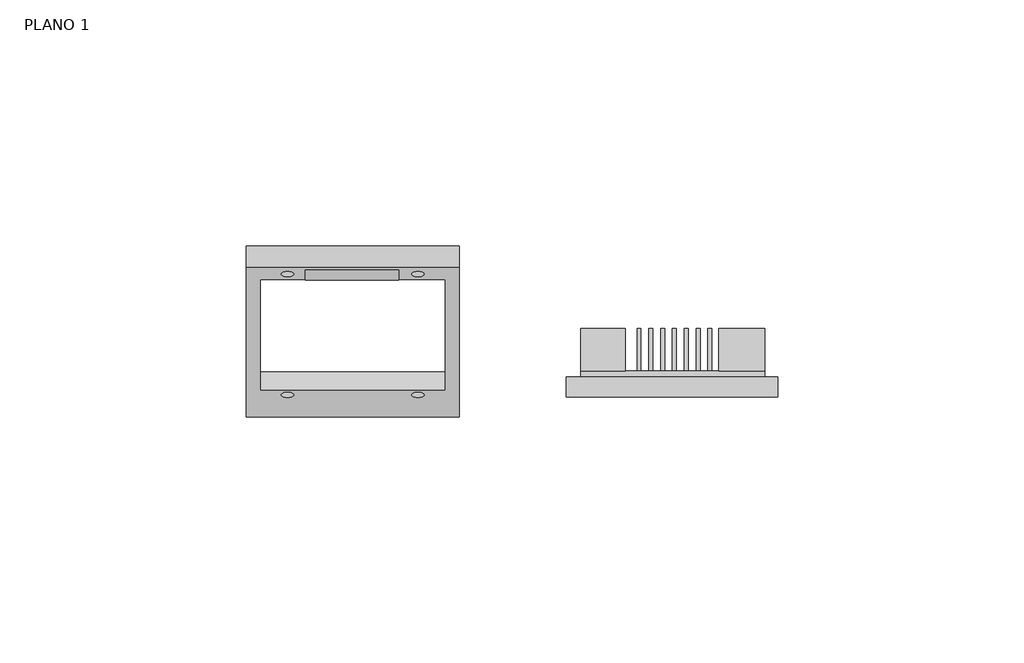
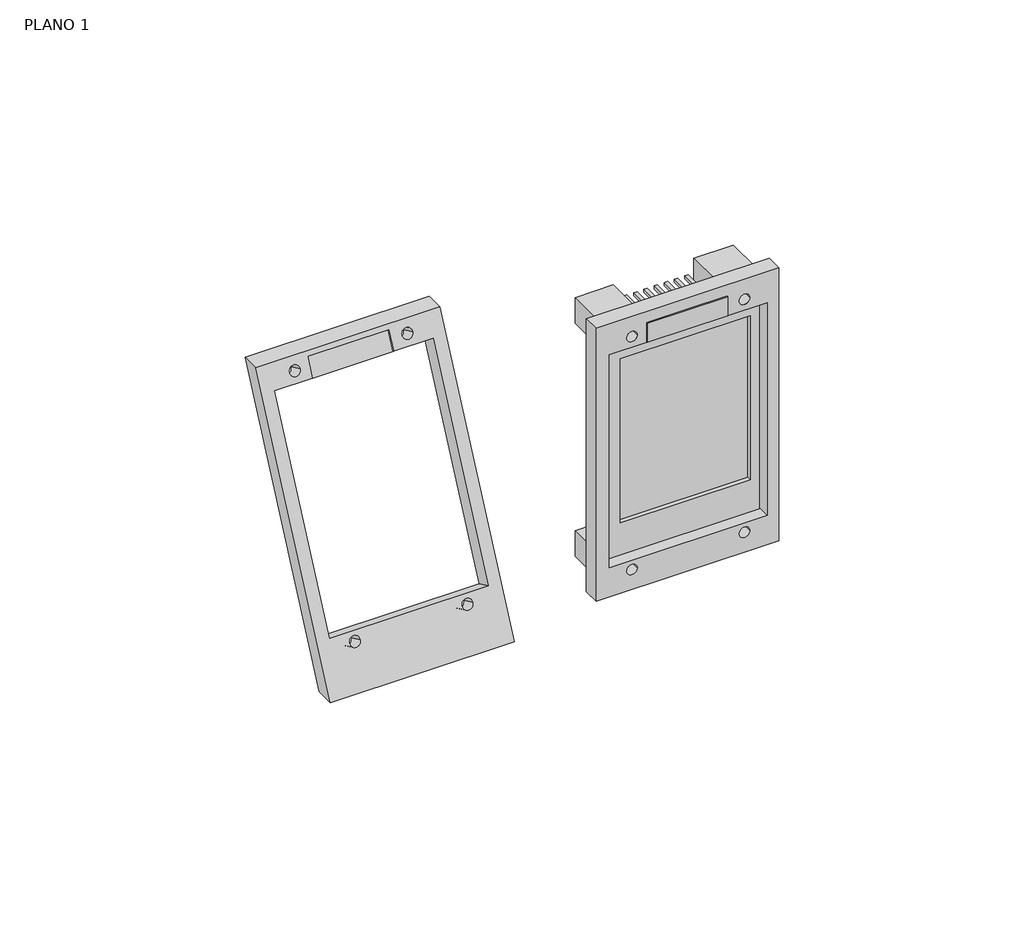
# One storey: 3 furniture elements, 2 proxies.
"""IFC4 building model written with IfcOpenShell, lengths in millimetres."""

import ifcopenshell
import ifcopenshell.guid

model = None  # the IFC model being written
_history = None  # IfcOwnerHistory: only IFC2X3 demands one
_inside = {}  # id of a spatial element -> (the spatial element, [elements in it])
_under = {}  # id of a project, library or spatial element -> (it, [spatial elements below it])
_declared = {}  # id of a project -> (the project, [libraries it declares])
_typed = {}  # id of a type object -> (the type object, [elements of that type])
_made_of = {}  # id of a material, layer set ... -> (it, [elements and type objects made of it])


def new_model(schema):
    """Start an empty IFC model of exactly this schema.

    Asked for "IFC4X3", IfcOpenShell would pick the latest addendum, in which some entities
    have other attributes; the version numbers below select the first issue.
    IFC2X3 requires an IfcOwnerHistory on every rooted entity: one is made here for all.
    """
    global model, _history
    if schema == "IFC4X3":
        model = ifcopenshell.file(schema_version=(4, 3, 0, 0))
    else:
        model = ifcopenshell.file(schema=schema)
    _inside.clear()
    _under.clear()
    _declared.clear()
    _typed.clear()
    _made_of.clear()
    _history = None
    if model.schema == "IFC2X3":
        org = make("IfcOrganization", Name="unknown")
        user = make(
            "IfcPersonAndOrganization",
            ThePerson=make("IfcPerson", FamilyName="unknown"),
            TheOrganization=org,
        )
        app = make(
            "IfcApplication",
            ApplicationDeveloper=org,
            Version="unknown",
            ApplicationFullName="unknown",
            ApplicationIdentifier="unknown",
        )
        _history = make(
            "IfcOwnerHistory",
            OwningUser=user,
            OwningApplication=app,
            ChangeAction="ADDED",
            CreationDate=0,
        )
    return model


def make(cls, **values):
    """One entity of the class cls with the attributes given. An attribute that is None is left unset."""
    return model.create_entity(
        cls, **{name: value for name, value in values.items() if value is not None}
    )


def rooted(cls, **values):
    """An entity with a GlobalId (a new one), such as an element, a storey or a relation."""
    return make(cls, GlobalId=ifcopenshell.guid.new(), OwnerHistory=_history, **values)


def si_unit(unit_type, name, prefix=None):
    """IfcSIUnit, for example si_unit("LENGTHUNIT", "METRE", prefix="MILLI")."""
    return make("IfcSIUnit", UnitType=unit_type, Prefix=prefix, Name=name)


def assignment(units):
    """IfcUnitAssignment: the units of a project."""
    return None if units is None else make("IfcUnitAssignment", Units=units)


def point(xyz):
    """IfcCartesianPoint."""
    return None if xyz is None else make("IfcCartesianPoint", Coordinates=xyz)


def direction(xyz):
    """IfcDirection."""
    return None if xyz is None else make("IfcDirection", DirectionRatios=xyz)


def frame(location, z_axis=None, x_axis=None):
    """IfcAxis2Placement3D, a coordinate frame: its origin and axes. An axis left out is left unset."""
    return make(
        "IfcAxis2Placement3D",
        Location=point(location),
        Axis=direction(z_axis),
        RefDirection=direction(x_axis),
    )


def frame_2d(location, x_axis=None):
    """IfcAxis2Placement2D, a coordinate frame in the plane: its origin and x axis."""
    return make(
        "IfcAxis2Placement2D", Location=point(location), RefDirection=direction(x_axis)
    )


def origin():
    """The frame at (0, 0, 0) with its axes left unset."""
    return frame((0.0, 0.0, 0.0))


def place(relative_to, where):
    """IfcLocalPlacement: puts the frame where relative to a parent placement (None: the world)."""
    return make(
        "IfcLocalPlacement", PlacementRelTo=relative_to, RelativePlacement=where
    )


def context(
    kind, dimensions, precision=None, world=None, true_north=None, identifier=None
):
    """IfcGeometricRepresentationContext, for example the 3D "Model" context."""
    return make(
        "IfcGeometricRepresentationContext",
        ContextIdentifier=identifier,
        ContextType=kind,
        CoordinateSpaceDimension=dimensions,
        Precision=precision,
        WorldCoordinateSystem=world,
        TrueNorth=true_north,
    )


def project(units=None, contexts=None):
    """IfcProject with its units and contexts."""
    return rooted(
        "IfcProject",
        Name="project",
        RepresentationContexts=contexts,
        UnitsInContext=assignment(units),
    )


def spatial(cls, under=None, at=None, **own):
    """A site, building, storey or space (cls), placed at a placement, below another one or the project."""
    s = rooted(cls, ObjectPlacement=at, **own)
    if under is not None:
        _under.setdefault(under.id(), (under, []))[1].append(s)
    return s


def polyline(points):
    """IfcPolyline through the points."""
    return make("IfcPolyline", Points=[point(p) for p in points])


def circle_curve(where, radius):
    """IfcCircle in the frame where."""
    return make("IfcCircle", Position=where, Radius=radius)


def trimmed(basis, trim1, trim2, sense, master):
    """IfcTrimmedCurve: the piece of a basis curve between two trims."""
    return make(
        "IfcTrimmedCurve",
        BasisCurve=basis,
        Trim1=trim1,
        Trim2=trim2,
        SenseAgreement=sense,
        MasterRepresentation=master,
    )


def segment(curve, same_sense, transition):
    """IfcCompositeCurveSegment."""
    return make(
        "IfcCompositeCurveSegment",
        Transition=transition,
        SameSense=same_sense,
        ParentCurve=curve,
    )


def composite_curve(segments, self_intersect=None):
    """IfcCompositeCurve: segments joined end to end."""
    return make("IfcCompositeCurve", Segments=segments, SelfIntersect=self_intersect)


def outline(outer, holes=None, kind="AREA"):
    """IfcArbitraryClosedProfileDef: a profile drawn as a closed curve; with holes, ...WithVoids."""
    if holes is None:
        return make("IfcArbitraryClosedProfileDef", ProfileType=kind, OuterCurve=outer)
    return make(
        "IfcArbitraryProfileDefWithVoids",
        ProfileType=kind,
        OuterCurve=outer,
        InnerCurves=holes,
    )


def extrude(swept, where, along, depth):
    """IfcExtrudedAreaSolid: the profile swept, set in the frame where, extruded along a direction by depth."""
    return make(
        "IfcExtrudedAreaSolid",
        SweptArea=swept,
        Position=where,
        ExtrudedDirection=direction(along),
        Depth=depth,
    )


def shape(context_of_items, identifier, shape_type, items):
    """IfcShapeRepresentation: the items that make up one representation, for example the "Body"."""
    return make(
        "IfcShapeRepresentation",
        ContextOfItems=context_of_items,
        RepresentationIdentifier=identifier,
        RepresentationType=shape_type,
        Items=items,
    )


def source(mapping_origin, context_of_items, identifier, shape_type, items):
    """IfcRepresentationMap: a shape defined once, which mapped items show again and again."""
    return make(
        "IfcRepresentationMap",
        MappingOrigin=mapping_origin,
        MappedRepresentation=shape(context_of_items, identifier, shape_type, items),
    )


def transform(
    local_origin,
    x_axis=None,
    y_axis=None,
    z_axis=None,
    scale=None,
    scale2=None,
    scale3=None,
    uniform=True,
):
    """IfcCartesianTransformationOperator3D, or its non-uniform kind. x_axis, y_axis, z_axis: its Axis1, 2, 3."""
    if uniform:
        return make(
            "IfcCartesianTransformationOperator3D",
            Axis1=direction(x_axis),
            Axis2=direction(y_axis),
            LocalOrigin=point(local_origin),
            Scale=scale,
            Axis3=direction(z_axis),
        )
    return make(
        "IfcCartesianTransformationOperator3DnonUniform",
        Axis1=direction(x_axis),
        Axis2=direction(y_axis),
        LocalOrigin=point(local_origin),
        Scale=scale,
        Axis3=direction(z_axis),
        Scale2=scale2,
        Scale3=scale3,
    )


def mapped(mapping_source, mapping_target):
    """IfcMappedItem: shows the shape of a source again, moved by a transform."""
    return make(
        "IfcMappedItem", MappingSource=mapping_source, MappingTarget=mapping_target
    )


def made_of(thing, what):
    """Note that an element or type object is made of a material, layer set ...; save() writes the relation."""
    if what is not None:
        _made_of.setdefault(what.id(), (what, []))[1].append(thing)
    return thing


def element(
    cls,
    number,
    at=None,
    inside=None,
    cuts=None,
    type_object=None,
    material=None,
    context=None,
    identifier="Body",
    shape_type=None,
    held_by="IfcProductDefinitionShape",
    body=None,
    shapes=None,
    **own,
):
    """One element of the class cls, such as IfcWall. Its Tag is "e" and its number.

    at: its placement. inside: the storey or other place that contains it. cuts: it is an
    opening in that element (IfcRelVoidsElement). A single representation is given by context,
    identifier, shape_type and body (its items); several are given by shapes. held_by: the class
    of the entity that holds the representations. save() writes the other relations.
    """
    e = rooted(cls, Tag="e%d" % number, ObjectPlacement=at, **own)
    if body is not None:
        shapes = [shape(context, identifier, shape_type, body)]
    if shapes is not None:
        e.Representation = make(held_by, Representations=shapes)
    if inside is not None:
        _inside.setdefault(inside.id(), (inside, []))[1].append(e)
    if cuts is not None:
        rooted(
            "IfcRelVoidsElement", RelatingBuildingElement=cuts, RelatedOpeningElement=e
        )
    if type_object is not None:
        _typed.setdefault(type_object.id(), (type_object, []))[1].append(e)
    return made_of(e, material)


def aggregate(whole, parts):
    """IfcRelAggregates: a whole, such as a stair, and the parts it consists of."""
    return rooted("IfcRelAggregates", RelatingObject=whole, RelatedObjects=parts)


def save(model, path):
    """Write the relations noted so far, then the file.

    IfcRelAggregates (storeys below a building ...), IfcRelContainedInSpatialStructure (elements
    in a storey), IfcRelDefinesByType, IfcRelAssociatesMaterial and IfcRelDeclares: one each for
    every whole, place, type object, material and project.
    """
    for whole, parts in _under.values():
        aggregate(whole, parts)
    for where, things in _inside.values():
        rooted(
            "IfcRelContainedInSpatialStructure",
            RelatedElements=things,
            RelatingStructure=where,
        )
    for kind, things in _typed.values():
        rooted("IfcRelDefinesByType", RelatedObjects=things, RelatingType=kind)
    for what, things in _made_of.values():
        rooted("IfcRelAssociatesMaterial", RelatedObjects=things, RelatingMaterial=what)
    for by, libraries in _declared.values():
        rooted("IfcRelDeclares", RelatingContext=by, RelatedDefinitions=libraries)
    model.write(path)


def plane_surface(at):
    """IfcPlane: the flat surface through the origin of the frame at, square to its z axis."""
    return make("IfcPlane", Position=at)


def revolved_surface(curve, axis_point, axis_direction):
    """IfcSurfaceOfRevolution: the curve turned about the line through axis_point along axis_direction."""
    return make(
        "IfcSurfaceOfRevolution",
        SweptCurve=make("IfcArbitraryOpenProfileDef", ProfileType="CURVE", Curve=curve),
        AxisPosition=make("IfcAxis1Placement", Location=point(axis_point), Axis=direction(axis_direction)),
    )


def advanced_brep(points, edges, surfaces, faces):
    """IfcAdvancedBrep: a solid bounded by faces that lie on surfaces and meet in shared edges.

    An edge is (start, end): straight between two places in points (the first is 0);
    or (start, end, curve); or (start, end, curve, False) where it runs against its curve.
    A face is (place in surfaces, loops), or (place, loops, False) where it looks against
    its surface's normal. A loop lists edges by number (the first is 1), with a minus sign
    where the edge is run from its end to its start. The first loop is the outer one.
    """
    corners = [point(p) for p in points]
    vertices = [make("IfcVertexPoint", VertexGeometry=c) for c in corners]
    made = []
    for start, end, *more in edges:
        made.append(
            make(
                "IfcEdgeCurve",
                EdgeStart=vertices[start],
                EdgeEnd=vertices[end],
                EdgeGeometry=more[0] if more else make("IfcPolyline", Points=[corners[start], corners[end]]),
                SameSense=more[1] if len(more) > 1 else True,
            )
        )
    hull = []
    for where, loops, *sense in faces:
        bounds = []
        for j, loop in enumerate(loops):
            ring = [make("IfcOrientedEdge", EdgeElement=made[abs(k) - 1], Orientation=k > 0) for k in loop]
            bounds.append(
                make(
                    "IfcFaceOuterBound" if j == 0 else "IfcFaceBound",
                    Bound=make("IfcEdgeLoop", EdgeList=ring),
                    Orientation=True,
                )
            )
        hull.append(make("IfcAdvancedFace", Bounds=bounds, FaceSurface=surfaces[where], SameSense=sense[0] if sense else True))
    return make("IfcAdvancedBrep", Outer=make("IfcClosedShell", CfsFaces=hull))


def base2_base_c05baaad(model_context):
    return source(origin(), model_context, "Body", "SweptSolid", [
        extrude(outline(polyline([(2465.0719295, 1293.4498458), (2465.0719295, 1291.7192449), (2446.0719295, 1291.7192449), (2446.0719295, 1293.4498458), (2465.0719295, 1293.4498458)])), frame((0.0, 0.0, 60.3), z_axis=(0.0, 0.0, 1.0), x_axis=(1.0, 0.0, 0.0)), (0.0, 0.0, 1.0), 4.7),
        extrude(outline(polyline([(0.0, 2434.0719295), (0.0, 2477.0719295), (68.0, 2477.0719295), (68.0, 2434.0719295), (0.0, 2434.0719295)]), holes=[composite_curve([segment(trimmed(circle_curve(frame_2d((63.0, 2468.9719295)), 1.25), [point((63.0, 2467.7219295))], [point((63.0, 2470.2219295))], True, "CARTESIAN"), True, "CONTINUOUS"), segment(trimmed(circle_curve(frame_2d((63.0, 2468.9719295)), 1.25), [point((63.0, 2470.2219295))], [point((63.0, 2467.7219295))], True, "CARTESIAN"), True, "CONTINUOUS")], self_intersect=False), composite_curve([segment(trimmed(circle_curve(frame_2d((5.0, 2468.9719295)), 1.25), [point((5.0, 2470.2219295))], [point((5.0, 2467.7219295))], True, "CARTESIAN"), True, "CONTINUOUS"), segment(trimmed(circle_curve(frame_2d((5.0, 2468.9719295)), 1.25), [point((5.0, 2467.7219295))], [point((5.0, 2470.2219295))], True, "CARTESIAN"), True, "CONTINUOUS")], self_intersect=False), composite_curve([segment(trimmed(circle_curve(frame_2d((5.0, 2442.4719295)), 1.25), [point((5.0, 2443.7219295))], [point((5.0, 2441.2219295))], True, "CARTESIAN"), True, "CONTINUOUS"), segment(trimmed(circle_curve(frame_2d((5.0, 2442.4719295)), 1.25), [point((5.0, 2441.2219295))], [point((5.0, 2443.7219295))], True, "CARTESIAN"), True, "CONTINUOUS")], self_intersect=False), composite_curve([segment(trimmed(circle_curve(frame_2d((63.0, 2442.4719295)), 1.25), [point((63.0, 2443.7219295))], [point((63.0, 2441.2219295))], True, "CARTESIAN"), True, "CONTINUOUS"), segment(trimmed(circle_curve(frame_2d((63.0, 2442.4719295)), 1.25), [point((63.0, 2441.2219295))], [point((63.0, 2443.7219295))], True, "CARTESIAN"), True, "CONTINUOUS")], self_intersect=False), polyline([(7.3, 2474.3719295), (7.3, 2437.0719295), (60.3, 2437.0719295), (60.3, 2446.0719295), (65.0, 2446.0719295), (65.0, 2465.0719295), (60.3, 2465.0719295), (60.3, 2474.3719295), (7.3, 2474.3719295)])]), frame((0.0, 1291.7192449, 0.0), z_axis=(0.0, 1.0, 0.0), x_axis=(0.0, 0.0, 1.0)), (0.0, 0.0, 1.0), 4.0),
    ])


def base3_base_5e775e04(model_context):
    return source(origin(), model_context, "Body", "SweptSolid", [
        extrude(outline(polyline([(59.8, 2465.0719295), (59.8, 2474.3719295), (66.2, 2474.3719295), (66.2, 2465.0719295), (59.8, 2465.0719295)]), holes=[composite_curve([segment(trimmed(circle_curve(frame_2d((63.0, 2468.9719295)), 1.7), [point((63.0, 2467.2719295))], [point((63.0, 2470.6719295))], True, "CARTESIAN"), True, "CONTINUOUS"), segment(trimmed(circle_curve(frame_2d((63.0, 2468.9719295)), 1.7), [point((63.0, 2470.6719295))], [point((63.0, 2467.2719295))], True, "CARTESIAN"), True, "CONTINUOUS")], self_intersect=False)]), frame((0.0, 1296.9192449, 0.0), z_axis=(0.0, 1.0, 0.0), x_axis=(0.0, 0.0, 1.0)), (0.0, 0.0, 1.0), 8.6306009),
        extrude(outline(polyline([(59.8, 2437.0719295), (59.8, 2446.0719295), (66.2, 2446.0719295), (66.2, 2437.0719295), (59.8, 2437.0719295)]), holes=[composite_curve([segment(trimmed(circle_curve(frame_2d((63.0, 2442.4719295)), 1.7), [point((63.0, 2444.1719295))], [point((63.0, 2440.7719295))], True, "CARTESIAN"), True, "CONTINUOUS"), segment(trimmed(circle_curve(frame_2d((63.0, 2442.4719295)), 1.7), [point((63.0, 2440.7719295))], [point((63.0, 2444.1719295))], True, "CARTESIAN"), True, "CONTINUOUS")], self_intersect=False)]), frame((0.0, 1296.9192449, 0.0), z_axis=(0.0, 1.0, 0.0), x_axis=(0.0, 0.0, 1.0)), (0.0, 0.0, 1.0), 8.6306009),
        extrude(outline(polyline([(1.8, 2465.0719295), (1.8, 2474.3719295), (8.2, 2474.3719295), (8.2, 2465.0719295), (1.8, 2465.0719295)]), holes=[composite_curve([segment(trimmed(circle_curve(frame_2d((5.0, 2468.9719295)), 1.7), [point((5.0, 2470.6719295))], [point((5.0, 2467.2719295))], True, "CARTESIAN"), True, "CONTINUOUS"), segment(trimmed(circle_curve(frame_2d((5.0, 2468.9719295)), 1.7), [point((5.0, 2467.2719295))], [point((5.0, 2470.6719295))], True, "CARTESIAN"), True, "CONTINUOUS")], self_intersect=False)]), frame((0.0, 1296.9192449, 0.0), z_axis=(0.0, 1.0, 0.0), x_axis=(0.0, 0.0, 1.0)), (0.0, 0.0, 1.0), 8.6306009),
        extrude(outline(polyline([(1.8, 2446.0719295), (8.2, 2446.0719295), (8.2, 2437.0719295), (1.8, 2437.0719295), (1.8, 2446.0719295)]), holes=[composite_curve([segment(trimmed(circle_curve(frame_2d((5.0, 2442.4719295)), 1.7), [point((5.0, 2444.1719295))], [point((5.0, 2440.7719295))], True, "CARTESIAN"), True, "CONTINUOUS"), segment(trimmed(circle_curve(frame_2d((5.0, 2442.4719295)), 1.7), [point((5.0, 2440.7719295))], [point((5.0, 2444.1719295))], True, "CARTESIAN"), True, "CONTINUOUS")], self_intersect=False)]), frame((0.0, 1296.9192449, 0.0), z_axis=(0.0, 1.0, 0.0), x_axis=(0.0, 0.0, 1.0)), (0.0, 0.0, 1.0), 8.6306009),
    ])


def furniture_6c0b4a62(model_context):
    return source(origin(), model_context, "Body", "AdvancedBrep", [
        advanced_brep(
        [(2369.0719295, 1292.0509228, 0.0), (2369.0719295, 1322.3609206, 65.0), (2412.3719295, 1322.3609206, 65.0), (2412.3719295, 1292.0509228, 0.0), (2402.7219295, 1320.2478293, 60.4684611), (2405.2219295, 1320.2478293, 60.4684611), (2409.3719295, 1296.7079921, 9.9871173), (2409.3719295, 1319.10676, 58.02143), (2400.0719295, 1319.10676, 58.02143), (2400.0719295, 1321.0930658, 62.2810766), (2381.0719295, 1321.0930658, 62.2810766), (2381.0719295, 1319.10676, 58.02143), (2372.0719295, 1319.10676, 58.02143), (2372.0719295, 1296.7079921, 9.9871173), (2405.2219295, 1295.7359701, 7.9026094), (2402.7219295, 1295.7359701, 7.9026094), (2378.7219295, 1295.7359701, 7.9026094), (2376.2219295, 1295.7359701, 7.9026094), (2378.7219295, 1320.2478293, 60.4684611), (2376.2219295, 1320.2478293, 60.4684611), (2412.3719295, 1287.6374112, 0.0), (2412.3719295, 1317.9474089, 65.0), (2369.0719295, 1317.9474089, 65.0), (2369.0719295, 1287.6374112, 0.0), (2402.7219295, 1316.6225981, 62.1589341), (2405.2219295, 1316.6225981, 62.1589341), (2409.3719295, 1293.082761, 11.6775904), (2372.0719295, 1293.082761, 11.6775904), (2372.0719295, 1315.4815288, 59.7119031), (2381.0719295, 1315.4815288, 59.7119031), (2381.0719295, 1317.4678347, 63.9715497), (2400.0719295, 1317.4678347, 63.9715497), (2400.0719295, 1315.4815288, 59.7119031), (2409.3719295, 1315.4815288, 59.7119031), (2405.2219295, 1292.110739, 9.5930825), (2402.7219295, 1292.110739, 9.5930825), (2378.7219295, 1292.110739, 9.5930825), (2376.2219295, 1292.110739, 9.5930825), (2378.7219295, 1316.6225981, 62.1589341), (2376.2219295, 1316.6225981, 62.1589341)],
        [
            (0, 1),
            (1, 2),
            (2, 3),
            (3, 0),
            (4, 5, circle_curve(frame((2403.9719295, 1320.2478293, 60.4684611), z_axis=(0.0, -0.9063077870366535, 0.4226182617406919), x_axis=(-1.0, 0.0, 0.0)), 1.25)),
            (5, 4, circle_curve(frame((2403.9719295, 1320.2478293, 60.4684611), z_axis=(0.0, -0.9063077870366535, 0.4226182617406919), x_axis=(-1.0, 0.0, 0.0)), 1.25)),
            (6, 7),
            (7, 8),
            (8, 9),
            (9, 10),
            (10, 11),
            (11, 12),
            (12, 13),
            (13, 6),
            (14, 15, circle_curve(frame((2403.9719295, 1295.7359701, 7.9026094), z_axis=(0.0, -0.9063077870366535, 0.4226182617406919), x_axis=(-1.0, 0.0, 0.0)), 1.25)),
            (15, 14, circle_curve(frame((2403.9719295, 1295.7359701, 7.9026094), z_axis=(0.0, -0.9063077870366535, 0.4226182617406919), x_axis=(-1.0, 0.0, 0.0)), 1.25)),
            (16, 17, circle_curve(frame((2377.4719295, 1295.7359701, 7.9026094), z_axis=(0.0, -0.9063077870366535, 0.4226182617406919), x_axis=(1.0, 0.0, 0.0)), 1.25)),
            (17, 16, circle_curve(frame((2377.4719295, 1295.7359701, 7.9026094), z_axis=(0.0, -0.9063077870366535, 0.4226182617406919), x_axis=(1.0, 0.0, 0.0)), 1.25)),
            (18, 19, circle_curve(frame((2377.4719295, 1320.2478293, 60.4684611), z_axis=(0.0, -0.9063077870366535, 0.4226182617406919), x_axis=(1.0, 0.0, 0.0)), 1.25)),
            (19, 18, circle_curve(frame((2377.4719295, 1320.2478293, 60.4684611), z_axis=(0.0, -0.9063077870366535, 0.4226182617406919), x_axis=(1.0, 0.0, 0.0)), 1.25)),
            (20, 21),
            (21, 22),
            (22, 23),
            (23, 20),
            (24, 25, circle_curve(frame((2403.9719295, 1316.6225981, 62.1589341), z_axis=(0.0, 0.9063077870366535, -0.4226182617406919), x_axis=(-1.0, 0.0, 0.0)), 1.25)),
            (25, 24, circle_curve(frame((2403.9719295, 1316.6225981, 62.1589341), z_axis=(0.0, 0.9063077870366535, -0.4226182617406919), x_axis=(-1.0, 0.0, 0.0)), 1.25)),
            (26, 27),
            (27, 28),
            (28, 29),
            (29, 30),
            (30, 31),
            (31, 32),
            (32, 33),
            (33, 26),
            (34, 35, circle_curve(frame((2403.9719295, 1292.110739, 9.5930825), z_axis=(0.0, 0.9063077870366535, -0.4226182617406919), x_axis=(-1.0, 0.0, 0.0)), 1.25)),
            (35, 34, circle_curve(frame((2403.9719295, 1292.110739, 9.5930825), z_axis=(0.0, 0.9063077870366535, -0.4226182617406919), x_axis=(-1.0, 0.0, 0.0)), 1.25)),
            (36, 37, circle_curve(frame((2377.4719295, 1292.110739, 9.5930825), z_axis=(0.0, 0.9063077870366535, -0.4226182617406919), x_axis=(1.0, 0.0, 0.0)), 1.25)),
            (37, 36, circle_curve(frame((2377.4719295, 1292.110739, 9.5930825), z_axis=(0.0, 0.9063077870366535, -0.4226182617406919), x_axis=(1.0, 0.0, 0.0)), 1.25)),
            (38, 39, circle_curve(frame((2377.4719295, 1316.6225981, 62.1589341), z_axis=(0.0, 0.9063077870366535, -0.4226182617406919), x_axis=(1.0, 0.0, 0.0)), 1.25)),
            (39, 38, circle_curve(frame((2377.4719295, 1316.6225981, 62.1589341), z_axis=(0.0, 0.9063077870366535, -0.4226182617406919), x_axis=(1.0, 0.0, 0.0)), 1.25)),
            (0, 23),
            (22, 1),
            (2, 21),
            (20, 3),
            (4, 24),
            (25, 5),
            (6, 26),
            (33, 7),
            (32, 8),
            (31, 9),
            (30, 10),
            (29, 11),
            (28, 12),
            (27, 13),
            (14, 34),
            (35, 15),
            (16, 36),
            (37, 17),
            (18, 38),
            (39, 19),
        ],
        [
            plane_surface(frame((2369.0719295, 1293.6228788, 3.3710705), z_axis=(0.0, 0.9063077870366535, -0.4226182617406919), x_axis=(0.0, 0.4226182617406919, 0.9063077870366535))),
            plane_surface(frame((2369.0719295, 1289.9976477, 5.0615435), z_axis=(0.0, -0.9063077870366535, 0.4226182617406919), x_axis=(0.0, -0.4226182617406919, -0.9063077870366535))),
            plane_surface(frame((2369.0719295, 1290.6199639, -3.0687014), z_axis=(-1.0, 0.0, 0.0), x_axis=(0.0, -0.9063077870366527, 0.42261826174069356))),
            plane_surface(frame((2412.3719295, 1322.3609206, 65.0), z_axis=(1.0, 0.0, 0.0), x_axis=(0.0, -0.9063077870366535, 0.42261826174069184))),
            revolved_surface(polyline([(2402.7219295, 1316.6225981272491, 62.15893415843589), (2402.7219295, 1320.2478293, 60.4684611)]), (2403.9719295, 1320.2478293, 60.4684611), (0.0, -0.9063077870366535, 0.4226182617406919)),
            plane_surface(frame((2409.3719295, 1296.7079921, 9.9871173), z_axis=(-1.0, 0.0, 0.0), x_axis=(0.0, -0.9063077870366532, 0.4226182617406927))),
            plane_surface(frame((2409.3719295, 1319.10676, 58.02143), z_axis=(0.0, -0.42261826174069184, -0.9063077870366535), x_axis=(0.0, -0.9063077870366535, 0.42261826174069184))),
            plane_surface(frame((2400.0719295, 1319.10676, 58.02143), z_axis=(-1.0, 0.0, 0.0), x_axis=(0.0, -0.9063077870366535, 0.42261826174069184))),
            plane_surface(frame((2400.0719295, 1321.0930658, 62.2810766), z_axis=(0.0, -0.42261826174069184, -0.9063077870366535), x_axis=(0.0, -0.9063077870366535, 0.42261826174069184))),
            plane_surface(frame((2381.0719295, 1321.0930658, 62.2810766), z_axis=(1.0, 0.0, 0.0), x_axis=(0.0, -0.9063077870366527, 0.42261826174069356))),
            plane_surface(frame((2381.0719295, 1319.10676, 58.02143), z_axis=(0.0, -0.42261826174069184, -0.9063077870366535), x_axis=(0.0, -0.9063077870366535, 0.42261826174069184))),
            plane_surface(frame((2372.0719295, 1319.10676, 58.02143), z_axis=(1.0, 0.0, 0.0), x_axis=(0.0, -0.9063077870366535, 0.42261826174069184))),
            plane_surface(frame((2372.0719295, 1296.7079921, 9.9871173), z_axis=(0.0, 0.4226182617406927, 0.9063077870366532), x_axis=(0.0, -0.9063077870366532, 0.4226182617406927))),
            revolved_surface(polyline([(2402.7219295, 1292.1107389710862, 9.593082437994347), (2402.7219295, 1295.7359701, 7.9026094)]), (2403.9719295, 1295.7359701, 7.9026094), (0.0, -0.9063077870366535, 0.4226182617406919)),
            revolved_surface(polyline([(2378.7219295, 1292.1107389710862, 9.593082437994347), (2378.7219295, 1295.7359701, 7.9026094)]), (2377.4719295, 1295.7359701, 7.9026094), (0.0, -0.9063077870366535, 0.4226182617406919)),
            revolved_surface(polyline([(2378.7219295, 1316.6225981272491, 62.15893415843589), (2378.7219295, 1320.2478293, 60.4684611)]), (2377.4719295, 1320.2478293, 60.4684611), (0.0, -0.9063077870366535, 0.4226182617406919)),
            plane_surface(frame((2418.7000554, 1312.6608189, 65.0), z_axis=(0.0, 0.0, 1.0), x_axis=(-1.0, 0.0, 0.0))),
            plane_surface(frame((2418.7000554, 1302.9468274, 0.0), z_axis=(0.0, 0.0, -1.0), x_axis=(-1.0, 0.0, 0.0))),
        ],
        [
            (0, [[1, 2, 3, 4], [5, 6], [7, 8, 9, 10, 11, 12, 13, 14], [15, 16], [17, 18], [19, 20]]),
            (1, [[21, 22, 23, 24], [25, 26], [27, 28, 29, 30, 31, 32, 33, 34], [35, 36], [37, 38], [39, 40]]),
            (2, [[-1, 41, -23, 42]]),
            (3, [[-3, 43, -21, 44]]),
            (4, [[-5, 45, -26, 46]]),
            (4, [[-6, -46, -25, -45]]),
            (5, [[-7, 47, -34, 48]]),
            (6, [[-8, -48, -33, 49]]),
            (7, [[-9, -49, -32, 50]]),
            (8, [[-10, -50, -31, 51]]),
            (9, [[-11, -51, -30, 52]]),
            (10, [[-12, -52, -29, 53]]),
            (11, [[-13, -53, -28, 54]]),
            (12, [[-14, -54, -27, -47]]),
            (13, [[-15, 55, -36, 56]]),
            (13, [[-16, -56, -35, -55]]),
            (14, [[-17, 57, -38, 58]]),
            (14, [[-18, -58, -37, -57]]),
            (15, [[-19, 59, -40, 60]]),
            (15, [[-20, -60, -39, -59]]),
            (16, [[-2, -42, -22, -43]]),
            (17, [[-4, -44, -24, -41]]),
        ],
    ),
    ])


def furniture_bc1ec6cb(model_context):
    return source(origin(), model_context, "Body", "SweptSolid", [
        extrude(outline(polyline([(0.0, -19.0), (0.0, 0.0), (2.0, 0.0), (2.0, -19.0), (0.0, -19.0)])), frame((2400.0719295, 1317.2941444, 58.8666666), z_axis=(0.0, 0.4226182617406868, 0.9063077870366559), x_axis=(0.0, -0.9063077870366559, 0.4226182617406868)), (0.0, 0.0, 1.0), 4.7),
    ])


def gmt020_02_gmt020_02_ca843257(model_context):
    return source(origin(), model_context, "Body", "SolidModel", [
        advanced_brep(
        [(18.3, -32.2, 62.0), (18.3, -31.0, 62.0), (-19.0, -31.0, 62.0), (-19.0, -32.2, 62.0), (18.3, -32.2, 0.0), (-19.0, -32.2, 0.0), (-19.0, -31.0, 0.0), (18.3, -31.0, 0.0), (-14.85, -31.0, 60.0), (-12.35, -31.0, 60.0), (-14.85, -31.0, 2.0), (-12.35, -31.0, 2.0), (14.15, -31.0, 60.0), (11.65, -31.0, 60.0), (14.15, -31.0, 2.0), (11.65, -31.0, 2.0), (-18.1, -32.2, 56.4), (17.4, -32.2, 56.4), (17.4, -32.2, 5.2), (-18.1, -32.2, 5.2), (-12.35, -32.2, 60.0), (-14.85, -32.2, 60.0), (-12.35, -32.2, 2.0), (-14.85, -32.2, 2.0), (11.65, -32.2, 60.0), (14.15, -32.2, 60.0), (11.65, -32.2, 2.0), (14.15, -32.2, 2.0), (17.4, -34.4693991, 56.4), (-18.1, -34.4693991, 56.4), (17.4, -34.4693991, 5.2), (-18.1, -34.4693991, 5.2), (-15.3, -34.4693991, 54.0), (15.3, -34.4693991, 54.0), (15.3, -34.4693991, 13.2), (-15.3, -34.4693991, 13.2), (-15.3, -33.4693991, 54.0), (15.3, -33.4693991, 54.0), (15.3, -33.4693991, 13.2), (-15.3, -33.4693991, 13.2)],
        [
            (0, 1),
            (1, 2),
            (2, 3),
            (3, 0),
            (4, 5),
            (5, 6),
            (6, 7),
            (7, 4),
            (0, 4),
            (7, 1),
            (6, 2),
            (8, 9, circle_curve(frame((-13.6, -31.0, 60.0), z_axis=(0.0, -1.0, 0.0), x_axis=(1.0, 0.0, 0.0)), 1.25)),
            (9, 8, circle_curve(frame((-13.6, -31.0, 60.0), z_axis=(0.0, -1.0, 0.0), x_axis=(1.0, 0.0, 0.0)), 1.25)),
            (10, 11, circle_curve(frame((-13.6, -31.0, 2.0), z_axis=(0.0, -1.0, 0.0), x_axis=(1.0, 0.0, 0.0)), 1.25)),
            (11, 10, circle_curve(frame((-13.6, -31.0, 2.0), z_axis=(0.0, -1.0, 0.0), x_axis=(1.0, 0.0, 0.0)), 1.25)),
            (12, 13, circle_curve(frame((12.9, -31.0, 60.0), z_axis=(0.0, -1.0, 0.0), x_axis=(-1.0, 0.0, 0.0)), 1.25)),
            (13, 12, circle_curve(frame((12.9, -31.0, 60.0), z_axis=(0.0, -1.0, 0.0), x_axis=(-1.0, 0.0, 0.0)), 1.25)),
            (14, 15, circle_curve(frame((12.9, -31.0, 2.0), z_axis=(0.0, -1.0, 0.0), x_axis=(-1.0, 0.0, 0.0)), 1.25)),
            (15, 14, circle_curve(frame((12.9, -31.0, 2.0), z_axis=(0.0, -1.0, 0.0), x_axis=(-1.0, 0.0, 0.0)), 1.25)),
            (5, 3),
            (16, 17),
            (17, 18),
            (18, 19),
            (19, 16),
            (20, 21, circle_curve(frame((-13.6, -32.2, 60.0), z_axis=(0.0, 1.0, 0.0), x_axis=(1.0, 0.0, 0.0)), 1.25)),
            (21, 20, circle_curve(frame((-13.6, -32.2, 60.0), z_axis=(0.0, 1.0, 0.0), x_axis=(1.0, 0.0, 0.0)), 1.25)),
            (22, 23, circle_curve(frame((-13.6, -32.2, 2.0), z_axis=(0.0, 1.0, 0.0), x_axis=(1.0, 0.0, 0.0)), 1.25)),
            (23, 22, circle_curve(frame((-13.6, -32.2, 2.0), z_axis=(0.0, 1.0, 0.0), x_axis=(1.0, 0.0, 0.0)), 1.25)),
            (24, 25, circle_curve(frame((12.9, -32.2, 60.0), z_axis=(0.0, 1.0, 0.0), x_axis=(-1.0, 0.0, 0.0)), 1.25)),
            (25, 24, circle_curve(frame((12.9, -32.2, 60.0), z_axis=(0.0, 1.0, 0.0), x_axis=(-1.0, 0.0, 0.0)), 1.25)),
            (26, 27, circle_curve(frame((12.9, -32.2, 2.0), z_axis=(0.0, 1.0, 0.0), x_axis=(-1.0, 0.0, 0.0)), 1.25)),
            (27, 26, circle_curve(frame((12.9, -32.2, 2.0), z_axis=(0.0, 1.0, 0.0), x_axis=(-1.0, 0.0, 0.0)), 1.25)),
            (28, 17),
            (16, 29),
            (29, 28),
            (30, 31),
            (31, 19),
            (18, 30),
            (28, 30),
            (31, 29),
            (32, 33),
            (33, 34),
            (34, 35),
            (35, 32),
            (8, 21),
            (20, 9),
            (10, 23),
            (22, 11),
            (32, 36),
            (36, 37),
            (37, 33),
            (34, 38),
            (38, 39),
            (39, 35),
            (37, 38),
            (36, 39),
            (12, 25),
            (24, 13),
            (14, 27),
            (26, 15),
        ],
        [
            plane_surface(frame((18.3, -32.2, 62.0), z_axis=(0.0, 0.0, 1.0), x_axis=(0.0, 1.0, 0.0))),
            plane_surface(frame((18.3, -32.2, 0.0), z_axis=(0.0, 0.0, -1.0), x_axis=(0.0, -1.0, 0.0))),
            plane_surface(frame((18.3, -32.2, 62.0), z_axis=(1.0, 0.0, 0.0), x_axis=(0.0, 0.0, -1.0))),
            plane_surface(frame((18.3, -31.0, 62.0), z_axis=(0.0, 1.0, 0.0), x_axis=(0.0, 0.0, -1.0))),
            plane_surface(frame((-19.0, -31.0, 62.0), z_axis=(-1.0, 0.0, 0.0), x_axis=(0.0, 0.0, -1.0))),
            plane_surface(frame((-19.0, -32.2, 62.0), z_axis=(0.0, -1.0, 0.0), x_axis=(0.0, 0.0, -1.0))),
            plane_surface(frame((17.4, -33.4693991, 56.4), z_axis=(0.0, 0.0, 1.0), x_axis=(0.0, 1.0, 0.0))),
            plane_surface(frame((17.4, -33.4693991, 5.2), z_axis=(0.0, 0.0, -1.0), x_axis=(0.0, -1.0, 0.0))),
            plane_surface(frame((17.4, -34.4693991, 56.4), z_axis=(1.0, 0.0, 0.0), x_axis=(0.0, 0.0, -1.0))),
            plane_surface(frame((-18.1, -32.2693991, 56.4), z_axis=(-1.0, 0.0, 0.0), x_axis=(0.0, 0.0, -1.0))),
            plane_surface(frame((-18.1, -34.4693991, 56.4), z_axis=(0.0, -1.0, 0.0), x_axis=(0.0, 0.0, -1.0))),
            revolved_surface(polyline([(-12.35, -32.2, 60.0), (-12.35, -31.0, 60.0)]), (-13.6, -28.9796632, 60.0), (0.0, -1.0, 0.0)),
            revolved_surface(polyline([(-12.35, -32.2, 2.0), (-12.35, -31.0, 2.0)]), (-13.6, -28.9796632, 2.0), (0.0, -1.0, 0.0)),
            plane_surface(frame((15.3, -34.4, 54.0), z_axis=(0.0, 0.0, -1.0), x_axis=(0.0, 1.0, 0.0))),
            plane_surface(frame((15.3, -34.4, 13.2), z_axis=(0.0, 0.0, 1.0), x_axis=(0.0, -1.0, 0.0))),
            plane_surface(frame((15.3, -34.4693991, 54.0), z_axis=(-1.0, 0.0, 0.0), x_axis=(0.0, 0.0, -1.0))),
            plane_surface(frame((15.3, -33.4693991, 54.0), z_axis=(0.0, -1.0, 0.0), x_axis=(0.0, 0.0, -1.0))),
            plane_surface(frame((-15.3, -33.4693991, 54.0), z_axis=(1.0, 0.0, 0.0), x_axis=(0.0, 0.0, -1.0))),
            revolved_surface(polyline([(11.65, -32.2, 60.0), (11.65, -31.0, 60.0)]), (12.9, -31.0, 60.0), (0.0, -1.0, 0.0)),
            revolved_surface(polyline([(11.65, -32.2, 2.0), (11.65, -31.0, 2.0)]), (12.9, -31.0, 2.0), (0.0, -1.0, 0.0)),
        ],
        [
            (0, [[1, 2, 3, 4]]),
            (1, [[5, 6, 7, 8]]),
            (2, [[-1, 9, -8, 10]]),
            (3, [[-2, -10, -7, 11], [12, 13], [14, 15], [16, 17], [18, 19]]),
            (4, [[-3, -11, -6, 20]]),
            (5, [[-4, -20, -5, -9], [21, 22, 23, 24], [25, 26], [27, 28], [29, 30], [31, 32]]),
            (6, [[33, -21, 34, 35]]),
            (7, [[36, 37, -23, 38]]),
            (8, [[-33, 39, -38, -22]]),
            (9, [[-34, -24, -37, 40]]),
            (10, [[-35, -40, -36, -39], [41, 42, 43, 44]]),
            (11, [[45, -25, 46, -12]]),
            (11, [[-45, -13, -46, -26]]),
            (12, [[47, -27, 48, -14]]),
            (12, [[-47, -15, -48, -28]]),
            (13, [[49, 50, 51, -41]]),
            (14, [[52, 53, 54, -43]]),
            (15, [[-51, 55, -52, -42]]),
            (16, [[-50, 56, -53, -55]]),
            (17, [[-49, -44, -54, -56]]),
            (18, [[57, -29, 58, -16]]),
            (18, [[-57, -17, -58, -30]]),
            (19, [[59, -31, 60, -18]]),
            (19, [[-59, -19, -60, -32]]),
        ],
    ),
        extrude(outline(polyline([(-7.6, -33.6693991), (-7.6, -22.3693991), (-6.8, -22.3693991), (-6.8, -33.6693991), (-7.6, -33.6693991)])), frame((0.0, 0.0, 58.8), z_axis=(0.0, 0.0, 1.0), x_axis=(1.0, 0.0, 0.0)), (0.0, 0.0, 1.0), 0.8),
        extrude(outline(polyline([(6.8, -33.6693991), (6.8, -22.3693991), (7.6, -22.3693991), (7.6, -33.6693991), (6.8, -33.6693991)])), frame((0.0, 0.0, 58.8), z_axis=(0.0, 0.0, 1.0), x_axis=(1.0, 0.0, 0.0)), (0.0, 0.0, 1.0), 0.8),
        extrude(outline(polyline([(4.4, -33.6693991), (4.4, -22.3693991), (5.2, -22.3693991), (5.2, -33.6693991), (4.4, -33.6693991)])), frame((0.0, 0.0, 58.8), z_axis=(0.0, 0.0, 1.0), x_axis=(1.0, 0.0, 0.0)), (0.0, 0.0, 1.0), 0.8),
        extrude(outline(polyline([(2.0, -33.6693991), (2.0, -22.3693991), (2.8, -22.3693991), (2.8, -33.6693991), (2.0, -33.6693991)])), frame((0.0, 0.0, 58.8), z_axis=(0.0, 0.0, 1.0), x_axis=(1.0, 0.0, 0.0)), (0.0, 0.0, 1.0), 0.8),
        extrude(outline(polyline([(-0.4, -33.6693991), (-0.4, -22.3693991), (0.4, -22.3693991), (0.4, -33.6693991), (-0.4, -33.6693991)])), frame((0.0, 0.0, 58.8), z_axis=(0.0, 0.0, 1.0), x_axis=(1.0, 0.0, 0.0)), (0.0, 0.0, 1.0), 0.8),
        extrude(outline(polyline([(-2.8, -33.6693991), (-2.8, -22.3693991), (-2.0, -22.3693991), (-2.0, -33.6693991), (-2.8, -33.6693991)])), frame((0.0, 0.0, 58.8), z_axis=(0.0, 0.0, 1.0), x_axis=(1.0, 0.0, 0.0)), (0.0, 0.0, 1.0), 0.8),
        extrude(outline(polyline([(-5.2, -33.6693991), (-5.2, -22.3693991), (-4.4, -22.3693991), (-4.4, -33.6693991), (-5.2, -33.6693991)])), frame((0.0, 0.0, 58.8), z_axis=(0.0, 0.0, 1.0), x_axis=(1.0, 0.0, 0.0)), (0.0, 0.0, 1.0), 0.8),
    ])


model = new_model("IFC4")

# Units and contexts
model_context = context("Model", 3, world=origin())
ifc_project = project(units=[si_unit("LENGTHUNIT", "METRE", prefix="MILLI")], contexts=[model_context])

# Site, building, storey
site = spatial("IfcSite", under=ifc_project)
building = spatial("IfcBuilding", under=site)
storey = spatial("IfcBuildingStorey", under=building, Name="PLANO 1", Elevation=0.0)

# Proxies
placement = place(None, origin())
base2_base_shape = base2_base_c05baaad(model_context)
element("IfcBuildingElementProxy", 1, Name="BASE2 : BASE", ObjectType="BASE2 : BASE", at=placement, inside=storey, context=model_context, shape_type="MappedRepresentation", body=[
    mapped(base2_base_shape, transform((0.0, 0.0, 0.0), x_axis=(1.0, 0.0, 0.0), y_axis=(0.0, 1.0, 0.0), z_axis=(0.0, 0.0, 1.0))),
])
base3_base_shape = base3_base_5e775e04(model_context)
element("IfcBuildingElementProxy", 2, Name="BASE3 : BASE", ObjectType="BASE3 : BASE", at=placement, inside=storey, context=model_context, shape_type="MappedRepresentation", body=[
    mapped(base3_base_shape, transform((0.0, 0.0, 0.0), x_axis=(1.0, 0.0, 0.0), y_axis=(0.0, 1.0, 0.0), z_axis=(0.0, 0.0, 1.0))),
])

# Furniture
furniture_shape = furniture_6c0b4a62(model_context)
element("IfcFurniture", 3, ObjectType="MOLDURA TELA : MOLDURA TELA", at=placement, inside=storey, context=model_context, shape_type="MappedRepresentation", body=[
    mapped(furniture_shape, transform((0.0, 0.0, 0.0), x_axis=(1.0, 0.0, 0.0), y_axis=(0.0, 1.0, 0.0), z_axis=(0.0, 0.0, 1.0))),
])
furniture_2_shape = furniture_bc1ec6cb(model_context)
element("IfcFurniture", 4, ObjectType="MOLDURA TELA1 : MOLDURA TELA", at=placement, inside=storey, context=model_context, shape_type="MappedRepresentation", body=[
    mapped(furniture_2_shape, transform((0.0, 0.0, 0.0), x_axis=(1.0, 0.0, 0.0), y_axis=(0.0, 1.0, 0.0), z_axis=(0.0, 0.0, 1.0))),
])
gmt020_02_gmt020_02_shape = gmt020_02_gmt020_02_ca843257(model_context)
element("IfcFurniture", 5, ObjectType="GMT020-02 : GMT020-02", at=placement, inside=storey, context=model_context, shape_type="MappedRepresentation", body=[
    mapped(gmt020_02_gmt020_02_shape, transform((2456.0719295, 1327.9192449, 3.0), x_axis=(1.0, 0.0, 0.0), y_axis=(0.0, 1.0, 0.0), z_axis=(0.0, 0.0, 1.0))),
])

save(model, "model.ifc")

# Revit data of these elements
# Project information
#   Data de emissão do projeto = "Data de emissão"
#   Status do projeto = "Status do projeto"
#   Nome do cliente = "Proprietário"
#   Endereço do projeto = "Insira aqui o endereço"
#   Nome do projeto = "Nome do projeto"
#   Número do projeto = "0001"
# Type "MOLDURA TELA : MOLDURA TELA"
#   Height = 0
# Type "MOLDURA TELA1 : MOLDURA TELA"
#   Height = 0
# Type "GMT020-02 : GMT020-02"
#   Default Elevation = 0
# Element 1 (IfcBuildingElementProxy, "BASE2 : BASE")
#   Phase Created = Fase 1
#   Materials on its faces: ".BOX FUNDO"
# Element 2 (IfcBuildingElementProxy, "BASE3 : BASE")
#   Phase Created = Fase 1
#   Materials on its faces: ".BOX FUNDO"
# Element 3 (IfcFurniture, "MOLDURA TELA : MOLDURA TELA")
#   Phase Created = Fase 1
#   Materials on its faces: ".BOX FUNDO"
# Element 4 (IfcFurniture, "MOLDURA TELA1 : MOLDURA TELA")
#   Phase Created = Fase 1
#   Materials on its faces: ".BOX FUNDO"
# Element 5 (IfcFurniture, "GMT020-02 : GMT020-02")
#   Phase Created = Fase 1
#   Materials on its faces: ".TELA"
# Materials
#   ".BOX FUNDO": class "Vidro", colour RGB 236 240 239, transparency 0.15, Cost = 0
#   ".TELA": class "Vidro", colour RGB 128 128 255, transparency 0.5, Cost = 0
